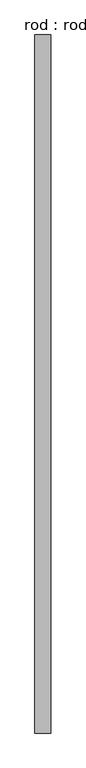
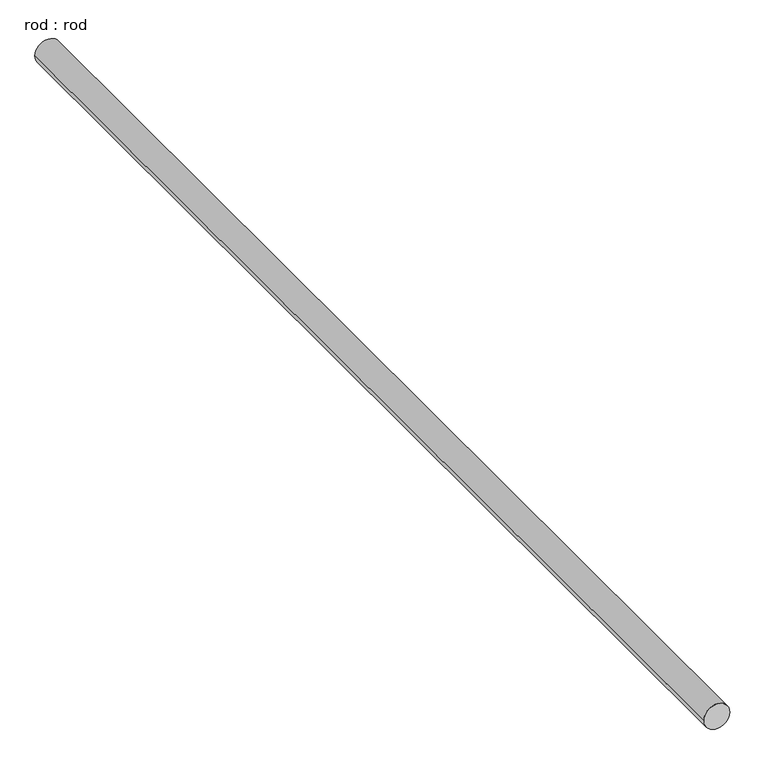
"""IFC4 building model written with IfcOpenShell, lengths in millimetres: proxy geometry, rod : rod."""

from ifc_helpers import new_model, si_unit, point, frame, frame_2d, origin, place, context, project, spatial, circle_curve, trimmed, segment, composite_curve, outline, extrude, source, transform, mapped, element, save


def rod_rod_14db28c1(model_context):
    return source(origin(), model_context, "Body", "SweptSolid", [
        extrude(outline(composite_curve([segment(trimmed(circle_curve(frame_2d((0.0108462, 0.0)), 200.0), [point((0.0108462, 200.0))], [point((0.0108462, -200.0))], False, "CARTESIAN"), True, "CONTINUOUS"), segment(trimmed(circle_curve(frame_2d((0.0108462, 0.0)), 200.0), [point((0.0108462, -200.0))], [point((0.0108462, 200.0))], False, "CARTESIAN"), True, "CONTINUOUS")], self_intersect=False)), frame((0.0, -4755.26383, 0.0), z_axis=(0.0, 1.0, 0.0), x_axis=(0.0, 0.0, 1.0)), (0.0, 0.0, 1.0), 17695.9848906),
    ])


if __name__ == "__main__":
    model = new_model("IFC4")
    model_context = context("Model", 3, world=origin())
    ifc_project = project(units=[si_unit("LENGTHUNIT", "METRE", prefix="MILLI")], contexts=[model_context])
    site = spatial("IfcSite", under=ifc_project)
    building = spatial("IfcBuilding", under=site)
    placement = place(None, origin())
    rod_rod_shape = rod_rod_14db28c1(model_context)
    element("IfcBuildingElementProxy", 1, Name="rod : rod", ObjectType="rod : rod", at=placement, inside=building, context=model_context, shape_type="MappedRepresentation", body=[
        mapped(rod_rod_shape, transform((0.0, 0.0, 0.0), x_axis=(1.0, 0.0, 0.0), y_axis=(0.0, 1.0, 0.0), z_axis=(0.0, 0.0, 1.0))),
    ])
    save(model, "model.ifc")

# Revit data of these elements
# Type "rod : rod"
#   Default Elevation = 0
